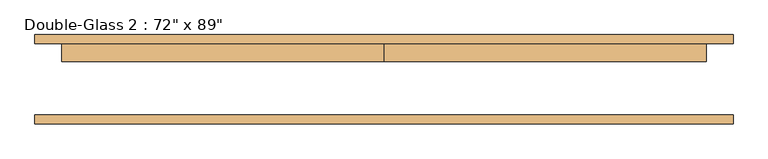
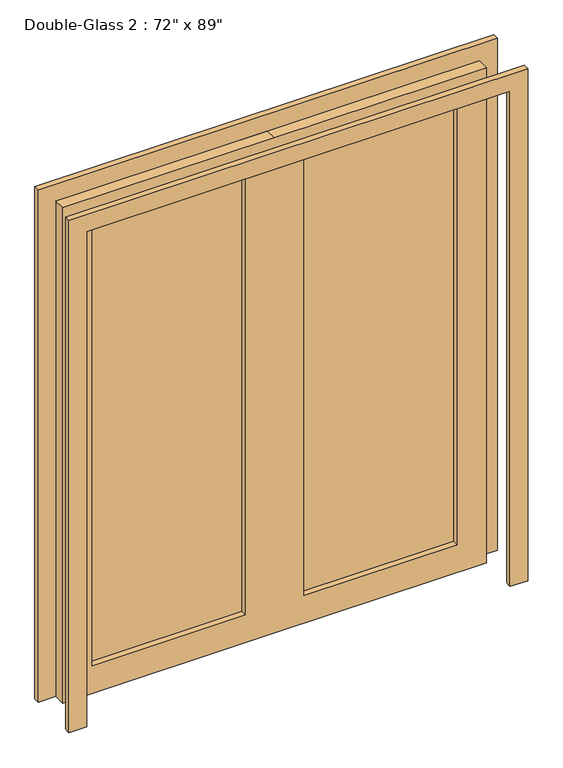
"""IFC4 building model written with IfcOpenShell, lengths in millimetres: door geometry."""

from ifc_helpers import new_model, si_unit, frame, origin, place, context, project, spatial, polyline, outline, extrude, source, transform, mapped, element, save


def door_5b8de96d(model_context):
    return source(origin(), model_context, "Body", "SweptSolid", [
        extrude(outline(polyline([(2260.6, 0.0), (2260.6, -914.4), (0.0, -914.4), (0.0, 0.0), (0.0, 914.4), (2260.6, 914.4), (2260.6, 0.0)]), holes=[polyline([(127.0, 787.4), (127.0, 127.0), (2184.4, 127.0), (2184.4, 787.4), (127.0, 787.4)]), polyline([(127.0, -787.4), (2184.4, -787.4), (2184.4, -127.0), (127.0, -127.0), (127.0, -787.4)])]), frame((0.0, 50.8, 0.0), z_axis=(0.0, 1.0, 0.0), x_axis=(0.0, 0.0, 1.0)), (0.0, 0.0, 1.0), 50.8),
        extrude(outline(polyline([(2260.6, -914.4), (2260.6, 914.4), (0.0, 914.4), (0.0, 990.6), (2336.8, 990.6), (2336.8, -990.6), (0.0, -990.6), (0.0, -914.4), (2260.6, -914.4)])), frame((0.0, -127.0, 0.0), z_axis=(0.0, 1.0, 0.0), x_axis=(0.0, 0.0, 1.0)), (0.0, 0.0, 1.0), 25.4),
        extrude(outline(polyline([(2260.6, -914.4), (2260.6, 914.4), (0.0, 914.4), (0.0, 990.6), (2336.8, 990.6), (2336.8, -990.6), (0.0, -990.6), (0.0, -914.4), (2260.6, -914.4)])), frame((0.0, 101.6, 0.0), z_axis=(0.0, 1.0, 0.0), x_axis=(0.0, 0.0, 1.0)), (0.0, 0.0, 1.0), 25.4),
        extrude(outline(polyline([(127.0, 82.55), (787.4, 82.55), (787.4, 76.2), (127.0, 76.2), (127.0, 82.55)])), frame((0.0, 0.0, 127.0), z_axis=(0.0, 0.0, 1.0), x_axis=(1.0, 0.0, 0.0)), (0.0, 0.0, 1.0), 2057.4),
        extrude(outline(polyline([(-787.4, 82.55), (-127.0, 82.55), (-127.0, 76.2), (-787.4, 76.2), (-787.4, 82.55)])), frame((0.0, 0.0, 127.0), z_axis=(0.0, 0.0, 1.0), x_axis=(1.0, 0.0, 0.0)), (0.0, 0.0, 1.0), 2057.4),
    ])


if __name__ == "__main__":
    model = new_model("IFC4")
    model_context = context("Model", 3, world=origin())
    ifc_project = project(units=[si_unit("LENGTHUNIT", "METRE", prefix="MILLI")], contexts=[model_context])
    site = spatial("IfcSite", under=ifc_project)
    building = spatial("IfcBuilding", under=site)
    placement = place(None, origin())
    door_shape = door_5b8de96d(model_context)
    element("IfcDoor", 1, ObjectType="Double-Glass 2 : 72\" x 89\"", at=placement, inside=building, context=model_context, shape_type="MappedRepresentation", body=[
        mapped(door_shape, transform((0.0, 0.0, 0.0), x_axis=(1.0, 0.0, 0.0), y_axis=(0.0, 1.0, 0.0), z_axis=(0.0, 0.0, 1.0))),
    ])
    save(model, "model.ifc")

# Revit data of these elements
# Type "Double-Glass 2 : 72\" x 89\""
#   Type Mark = "20"
#   Construction Type Id = "GSP4R"
#   Assembly Code = "C1020"
#   Analytic Construction = "1/8 in Pilkington single glazing"
#   Visual Light Transmittance = 0.9
#   Thickness = 0' - 2"
#   Solar Heat Gain Coefficient = 0.78
#   Heat Transfer Coefficient (U) = 3.6886 W/(m²·K)
#   Height = 7' - 5"
#   Muntin = 0' - 1"
#   Trim Projection Ext = 0' - 1"
#   Trim Projection Int = 0' - 1"
#   Trim Width = 0' - 3"
#   Width = 6' - 0"
#   Door Material = Aluminum
#   Frame Material = Aluminum
#   Thermal Resistance (R) = 0
#   Function = (empty or 0)
#   Wall Closure = (empty or 0)
# Element 1 (IfcDoor, "Double-Glass 2 : 72\" x 89\"")
#   Materials on its faces: "Aluminum", "Glass"
# Materials
#   "Aluminum": class "Metal", colour RGB 247 247 247, transparency 0, Description = "Aluminum 6061", Cost = 0
#   "Glass": class "Glass", colour RGB 218 227 224, transparency 0.85, Description = "Soda Lime Glass", Cost = 0
